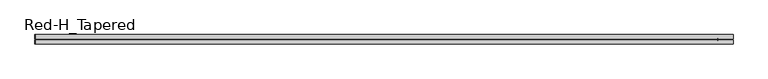
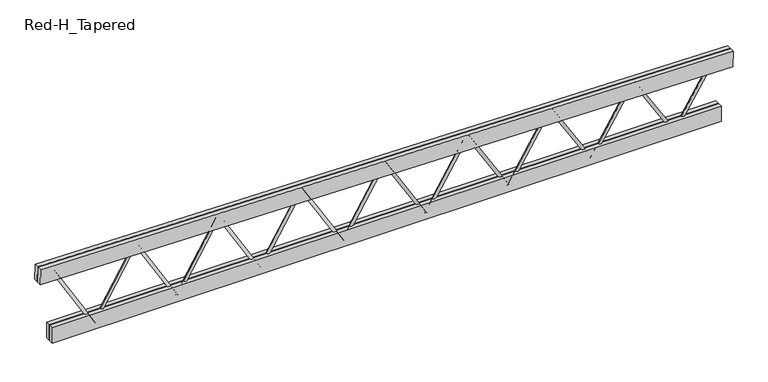
"""IFC4 building model written with IfcOpenShell, lengths in millimetres: beam geometry, Construction_Frames_RedBuilt_Openweb_Red-H_Tapered : Red-H_Tapered."""

from ifc_helpers import new_model, si_unit, point, frame, origin, origin_2d, place, context, project, spatial, polyline, circle_curve, trimmed, segment, composite_curve, outline, extrude, source, transform, mapped, element, save


def red_h_tapered_6d79e80b(model_context):
    return source(origin(), model_context, "Body", "SweptSolid", [
        extrude(outline(composite_curve([segment(trimmed(circle_curve(origin_2d(), 12.7), [point((0.0, 12.7))], [point((0.0, -12.7))], False, "CARTESIAN"), True, "CONTINUOUS"), segment(trimmed(circle_curve(origin_2d(), 12.7), [point((0.0, -12.7))], [point((0.0, 12.7))], False, "CARTESIAN"), True, "CONTINUOUS")], self_intersect=False)), frame((2526.107324, 0.0, -367.0101562), z_axis=(0.5255382750472374, 0.0, 0.8507699580147235), x_axis=(0.0, -1.0, 0.0)), (0.0, 0.0, 1.0), 686.6721074),
        extrude(outline(composite_curve([segment(trimmed(circle_curve(origin_2d(), 12.7), [point((0.0, -12.7))], [point((0.0, 12.6999999))], False, "CARTESIAN"), True, "CONTINUOUS"), segment(trimmed(circle_curve(origin_2d(), 12.7), [point((0.0, 12.6999999))], [point((0.0, -12.7))], False, "CARTESIAN"), True, "CONTINUOUS")], self_intersect=False)), frame((2526.107324, 0.0, -367.0101562), z_axis=(-0.5229651633515324, 0.0, 0.8523540566693545), x_axis=(0.0, -1.0, 0.0)), (0.0, 0.0, 1.0), 690.0506958),
        extrude(outline(composite_curve([segment(trimmed(circle_curve(origin_2d(), 12.7), [point((0.0, 12.7))], [point((0.0, -12.6999999))], False, "CARTESIAN"), True, "CONTINUOUS"), segment(trimmed(circle_curve(origin_2d(), 12.7), [point((0.0, -12.6999999))], [point((0.0, 12.7))], False, "CARTESIAN"), True, "CONTINUOUS")], self_intersect=False)), frame((1804.3623743, 0.0, -367.0101562), z_axis=(0.5229651633515339, 0.0, 0.8523540566693536), x_axis=(0.0, -1.0, 0.0)), (0.0, 0.0, 1.0), 690.0506958),
        extrude(outline(composite_curve([segment(trimmed(circle_curve(origin_2d(), 12.7), [point((0.0, -12.7000001))], [point((0.0, 12.6999999))], False, "CARTESIAN"), True, "CONTINUOUS"), segment(trimmed(circle_curve(origin_2d(), 12.7), [point((0.0, 12.6999999))], [point((0.0, -12.7000001))], False, "CARTESIAN"), True, "CONTINUOUS")], self_intersect=False)), frame((1804.3623743, 0.0, -367.0101562), z_axis=(-0.5204124432875953, 0.0, 0.8539150360963529), x_axis=(0.0, -1.0, 0.0)), (0.0, 0.0, 1.0), 693.4355231),
        extrude(outline(composite_curve([segment(trimmed(circle_curve(origin_2d(), 12.7), [point((0.0, 12.7))], [point((0.0, -12.7))], False, "CARTESIAN"), True, "CONTINUOUS"), segment(trimmed(circle_curve(origin_2d(), 12.7), [point((0.0, -12.7))], [point((0.0, 12.7))], False, "CARTESIAN"), True, "CONTINUOUS")], self_intersect=False)), frame((1082.6174246, 0.0, -367.0101562), z_axis=(0.5204124432875943, 0.0, 0.8539150360963534), x_axis=(0.0, -1.0, 0.0)), (0.0, 0.0, 1.0), 693.4355231),
        extrude(outline(composite_curve([segment(trimmed(circle_curve(origin_2d(), 12.7), [point((0.0, -12.7000001))], [point((0.0, 12.7))], False, "CARTESIAN"), True, "CONTINUOUS"), segment(trimmed(circle_curve(origin_2d(), 12.7), [point((0.0, 12.7))], [point((0.0, -12.7000001))], False, "CARTESIAN"), True, "CONTINUOUS")], self_intersect=False)), frame((1082.6174246, 0.0, -367.0101562), z_axis=(-0.5178799538342008, 0.0, 0.855453302884901), x_axis=(0.0, -1.0, 0.0)), (0.0, 0.0, 1.0), 696.8264985),
        extrude(outline(composite_curve([segment(trimmed(circle_curve(origin_2d(), 12.7), [point((0.0, 12.7))], [point((0.0, -12.7))], False, "CARTESIAN"), True, "CONTINUOUS"), segment(trimmed(circle_curve(origin_2d(), 12.7), [point((0.0, -12.7))], [point((0.0, 12.7))], False, "CARTESIAN"), True, "CONTINUOUS")], self_intersect=False)), frame((360.8724749, 0.0, -367.0101562), z_axis=(0.5178799538342008, 0.0, 0.855453302884901), x_axis=(0.0, -1.0, 0.0)), (0.0, 0.0, 1.0), 696.8264985),
        extrude(outline(composite_curve([segment(trimmed(circle_curve(origin_2d(), 12.7), [point((0.0, -12.7000001))], [point((0.0, 12.6999999))], False, "CARTESIAN"), True, "CONTINUOUS"), segment(trimmed(circle_curve(origin_2d(), 12.7), [point((0.0, 12.6999999))], [point((0.0, -12.7000001))], False, "CARTESIAN"), True, "CONTINUOUS")], self_intersect=False)), frame((360.8724749, 0.0, -367.0101562), z_axis=(-0.5153675335242818, 0.0, 0.856969255801571), x_axis=(0.0, -1.0, 0.0)), (0.0, 0.0, 1.0), 700.2235325),
        extrude(outline(composite_curve([segment(trimmed(circle_curve(origin_2d(), 12.7), [point((0.0, -12.6999999))], [point((0.0, 12.7000001))], False, "CARTESIAN"), True, "CONTINUOUS"), segment(trimmed(circle_curve(origin_2d(), 12.7), [point((0.0, 12.7000001))], [point((0.0, -12.6999999))], False, "CARTESIAN"), True, "CONTINUOUS")], self_intersect=False)), frame((-360.8724749, 0.0, -367.0101562), z_axis=(0.5153675335242504, 0.0, 0.8569692558015899), x_axis=(0.0, -1.0, 0.0)), (0.0, 0.0, 1.0), 700.2235325),
        extrude(outline(composite_curve([segment(trimmed(circle_curve(origin_2d(), 12.7), [point((0.0, 12.7))], [point((0.0, -12.7))], False, "CARTESIAN"), True, "CONTINUOUS"), segment(trimmed(circle_curve(origin_2d(), 12.7), [point((0.0, -12.7))], [point((0.0, 12.7))], False, "CARTESIAN"), True, "CONTINUOUS")], self_intersect=False)), frame((-360.8724749, 0.0, -367.0101562), z_axis=(-0.5128750205463383, 0.0, 0.8584632859357428), x_axis=(0.0, -1.0, 0.0)), (0.0, 0.0, 1.0), 703.6265375),
        extrude(outline(composite_curve([segment(trimmed(circle_curve(origin_2d(), 12.7), [point((0.0, -12.6999999))], [point((0.0, 12.7000001))], False, "CARTESIAN"), True, "CONTINUOUS"), segment(trimmed(circle_curve(origin_2d(), 12.7), [point((0.0, 12.7000001))], [point((0.0, -12.6999999))], False, "CARTESIAN"), True, "CONTINUOUS")], self_intersect=False)), frame((-1082.6174246, 0.0, -367.0101562), z_axis=(0.5128750205463365, 0.0, 0.858463285935744), x_axis=(0.0, -1.0, 0.0)), (0.0, 0.0, 1.0), 703.6265375),
        extrude(outline(composite_curve([segment(trimmed(circle_curve(origin_2d(), 12.7), [point((0.0, 12.7))], [point((0.0, -12.7))], False, "CARTESIAN"), True, "CONTINUOUS"), segment(trimmed(circle_curve(origin_2d(), 12.7), [point((0.0, -12.7))], [point((0.0, 12.7))], False, "CARTESIAN"), True, "CONTINUOUS")], self_intersect=False)), frame((-1082.6174246, 0.0, -367.0101562), z_axis=(-0.5104022528410607, 0.0, 0.8599357768431141), x_axis=(0.0, -1.0, 0.0)), (0.0, 0.0, 1.0), 707.0354272),
        extrude(outline(composite_curve([segment(trimmed(circle_curve(origin_2d(), 12.7), [point((0.0, -12.7))], [point((0.0, 12.7000001))], False, "CARTESIAN"), True, "CONTINUOUS"), segment(trimmed(circle_curve(origin_2d(), 12.7), [point((0.0, 12.7000001))], [point((0.0, -12.7))], False, "CARTESIAN"), True, "CONTINUOUS")], self_intersect=False)), frame((-1804.3623743, 0.0, -367.0101562), z_axis=(0.510402252841074, 0.0, 0.8599357768431061), x_axis=(0.0, -1.0, 0.0)), (0.0, 0.0, 1.0), 707.0354272),
        extrude(outline(composite_curve([segment(trimmed(circle_curve(origin_2d(), 12.7), [point((0.0, 12.6999999))], [point((0.0, -12.7))], False, "CARTESIAN"), True, "CONTINUOUS"), segment(trimmed(circle_curve(origin_2d(), 12.7), [point((0.0, -12.7))], [point((0.0, 12.6999999))], False, "CARTESIAN"), True, "CONTINUOUS")], self_intersect=False)), frame((-1804.3623743, 0.0, -367.0101562), z_axis=(-0.5079490681928376, 0.0, 0.8613871046875662), x_axis=(0.0, -1.0, 0.0)), (0.0, 0.0, 1.0), 710.4501169),
        extrude(outline(composite_curve([segment(trimmed(circle_curve(origin_2d(), 12.7), [point((0.0, -12.6999999))], [point((0.0, 12.7))], False, "CARTESIAN"), True, "CONTINUOUS"), segment(trimmed(circle_curve(origin_2d(), 12.7), [point((0.0, 12.7))], [point((0.0, -12.6999999))], False, "CARTESIAN"), True, "CONTINUOUS")], self_intersect=False)), frame((-2526.107324, 0.0, -367.0101562), z_axis=(0.5079490681928277, 0.0, 0.861387104687572), x_axis=(0.0, -1.0, 0.0)), (0.0, 0.0, 1.0), 710.4501169),
        extrude(outline(composite_curve([segment(trimmed(circle_curve(origin_2d(), 12.7), [point((0.0, 12.7))], [point((0.0, -12.7))], False, "CARTESIAN"), True, "CONTINUOUS"), segment(trimmed(circle_curve(origin_2d(), 12.7), [point((0.0, -12.7))], [point((0.0, 12.7))], False, "CARTESIAN"), True, "CONTINUOUS")], self_intersect=False)), frame((-2526.107324, 0.0, -367.0101562), z_axis=(-0.5055153043168177, 0.0, 0.8628176383810633), x_axis=(0.0, -1.0, 0.0)), (0.0, 0.0, 1.0), 713.8705234),
        extrude(outline(polyline([(-2912.3797989, -41.275), (-2912.3797989, -3.175), (2912.3797989, -3.175), (2912.3797989, -41.275), (-2912.3797989, -41.275)])), frame((0.0, 0.0, -386.0601562), z_axis=(0.0, 0.0, 1.0), x_axis=(1.0, 0.0, 0.0)), (0.0, 0.0, 1.0), 139.7),
        extrude(outline(polyline([(-2912.3797989, 3.175), (-2912.3797989, 41.275), (2912.3797989, 41.275), (2912.3797989, 3.175), (-2912.3797989, 3.175)])), frame((0.0, 0.0, -386.0601562), z_axis=(0.0, 0.0, 1.0), x_axis=(1.0, 0.0, 0.0)), (0.0, 0.0, 1.0), 139.7),
        extrude(outline(polyline([(0.0, -38.1), (0.0, 0.0), (6028.8157603, 0.0), (6028.8157603, -38.1), (0.0, -38.1)])), frame((-3016.3340788, -3.175, 185.4596828), z_axis=(0.016852397558582144, 0.0, 0.9998579882645973), x_axis=(0.9998579882645973, 0.0, -0.016852397558582144)), (0.0, 0.0, 1.0), 139.7),
        extrude(outline(polyline([(0.0, -38.1), (0.0, 0.0), (6028.8157603, 0.0), (6028.8157603, -38.1), (0.0, -38.1)])), frame((-3016.3340788, 41.275, 185.4596828), z_axis=(0.016852397558582144, 0.0, 0.9998579882645973), x_axis=(0.9998579882645973, 0.0, -0.016852397558582144)), (0.0, 0.0, 1.0), 139.7),
    ])


if __name__ == "__main__":
    model = new_model("IFC4")
    model_context = context("Model", 3, world=origin())
    ifc_project = project(units=[si_unit("LENGTHUNIT", "METRE", prefix="MILLI")], contexts=[model_context])
    site = spatial("IfcSite", under=ifc_project)
    building = spatial("IfcBuilding", under=site)
    placement = place(None, origin())
    red_h_tapered_shape = red_h_tapered_6d79e80b(model_context)
    element("IfcBeam", 1, ObjectType="Construction_Frames_RedBuilt_Openweb_Red-H_Tapered : Red-H_Tapered", at=placement, inside=building, context=model_context, shape_type="MappedRepresentation", body=[
        mapped(red_h_tapered_shape, transform((0.0, 0.0, 0.0), x_axis=(1.0, 0.0, 0.0), y_axis=(0.0, 1.0, 0.0), z_axis=(0.0, 0.0, 1.0))),
    ])
    save(model, "model.ifc")

# Revit data of these elements
# Type "Construction_Frames_RedBuilt_Openweb_Red-H_Tapered : Red-H_Tapered"
#   Youtube clip = ""
#   Weight Net (Kg) = "0"
#   Webs = "Up to 2\" diameter tubular steel"
#   Uniformat II Description = ""
#   Uniformat II Code = ""
#   Uniclass 2015 Name = "Softwood trusses"
#   Uniclass 2015 Code = "Pr_20_85_90_81"
#   Uniclass 2.0 Description = "Structural Framing Systems"
#   Uniclass 2.0 Code = "SS-15-10-75"
#   Uniclass 1.4 Description = "Trusses"
#   Uniclass 1.4 Code = "L3523"
#   UNSPSC Code = "30103606"
#   Technical description = "http://www.redbuilt.com/reference/literature-and-other-resources"
#   Region South America = "None"
#   Region Oceania = "None"
#   Region North America = "US"
#   Region Middle East = "None"
#   Region Europe = "None"
#   Region Asia = "None"
#   Region Antarctica = "None"
#   Region Africa = "None"
#   QR code = "http://bimobject.com/redbuilt/product/redbuilt-0003"
#   Product url = "http://www.redbuilt.com/products/default.aspx?id=2"
#   Product group = "Wood Trusses"
#   Product family = "Construction"
#   Product data url = "https://bimobject.com/redbuilt/product/redbuilt-0003"
#   Product certification = ""
#   Product SKU = "redbuilt-0003"
#   Product Page URL = "http://www.redbuilt.com/commercial-systems/red-m-red-h-open-web-trusses"
#   Product Guid = "2c5793f2-6ffb-4665-b825-cf90c048e711"
#   Product Documentation Link = "http://www.redbuilt.com/documents/OW_Guide_2017_07_LowRes_wLinks.pdf"
#   OmniClass Description = "Wood Trusses"
#   OmniClass Code = "23-13 35 19 13 17"
#   NBS Reference Description = ""
#   NBS Reference Code = ""
#   Material secondary = "Steel"
#   Material main = "CHARRED WOOD"
#   Masterformat 2014 Description = "Metal-Web Wood Joists"
#   Masterformat 2014 Code = "06 17 36"
#   Manufacturer name = "RedBuilt"
#   Manufacturer country = "United States"
#   Installation instructions = "http://www.redbuilt.com/documents/Installation_Sheets_Open-Web.pdf"
#   IFC Classification = ""
#   EAN code = ""
#   Design country = "United States"
#   Product Information = "http://redbuilt.com/products/default.aspx?id=2"
#   Model = "Red-H-Tapered"
#   Manufacturer URL = "http://redbuilt.com/"
#   Manufacturer = "RedBuilt™"
#   Description = "Open Web Truss"
#   Date of publishing = "8/17/2010"
#   Contact us = "http://redbuilt.com/contact/"
#   Chords = "Double 1½\" x 5½\" MSR lumber"
#   COBIe Type Category = ""
#   Brand url = "http://www.redbuilt.com"
#   BIMobject main category code = "construction"
#   BIMobject main category = "Construction"
#   BIMobject category code = "construction-frames-trusses"
#   BIMobject category = "Frames & Trusses"
#   Web Radius = 0' - 0 1/2"
#   Web Layout Offset Start [instance default] = 0' - 5"
#   Web Layout Offset End [instance default] = 0' - 5"
#   Web Diameter = 0' - 1"
#   TotalLength [instance default] = 20' - 0"
#   Span Minimum = 4' - 0"
#   Span Maximum = 70' - 0"
#   Span Limit [instance default] = 20' - 0"
#   Nominal width = 0' - 0"
#   Nominal height = 0' - 0"
#   Inner Depth Top [instance default] = 0' - 2.76372"
#   Depth Start [instance default] = 6' - 0"
#   Top Chord Length [instance default] = 20' - 1.19701"
#   TC Extension Start Aux [instance default] = 0' - 0"
#   TC Extension End Aux [instance default] = 0' - 0"
#   T-B Chord Length Difference L [instance default] = 0' - 4"
#   T-B Chord Length Difference [instance default] = 0' - 4"
#   Height 2 [instance default] = 6' - 0"
#   Depth Minimum at Wall = 2' - 0"
#   Depth Maximum at Wall = 6' - 0"
#   Depth Lower End [instance default] = 2' - 0"
#   Depth Higher End [instance default] = 6' - 0"
#   Depth End [instance default] = 2' - 0"
#   Depth 2 [instance default] = 2' - 0"
#   Chord Width = 0' - 3 1/4"
#   Chord Thickness = 0' - 1 1/2"
#   Chord Depth = 0' - 5 1/2"
#   Offset Start [instance default] = 0' - 0"
#   TC Extension Start [instance default] = 0' - 0"
#   End Panel = 0' - 5"
#   Offset End [instance default] = 0' - 0"
#   TC Extension End [instance default] = 0' - 0"
#   Length [instance default] = 20' - 0"
#   Angle [instance default] = 5.71059°
#   Span Limit Warning [instance default] = no
#   Edition number = 1
#   Top Bearing Start [instance default] = yes
#   Top Bearing End [instance default] = yes
#   Bottom Bearing Start [instance default] = no
#   Bottom Bearing End [instance default] = no
#   8 Panels [instance default] = yes
#   16 Panels [instance default] = no
#   12 Panels [instance default] = no
#   Web Material = RedBuilt-Steel, Galvanized
#   Clip Material = RedBuilt-Steel, Galvanized
#   Chords Material = WOOD-OAKFIRE
#   URL = ""
#   Assembly Code = ""
# Element 1 (IfcBeam, "Construction_Frames_RedBuilt_Openweb_Red-H_Tapered : Red-H_Tapered")
#   TotalLength = 19' - 9.32124"
#   Span Limit = 19' - 9.32124"
#   Inner Depth Top = 0' - 2.75039"
#   Depth Start = 5' - 0"
#   Top Chord Length = 19' - 9.35495"
#   Height 2 = 5' - 0"
#   Depth Higher End = 5' - 0"
#   Depth 2 = 0' - 4"
#   Angle = 0.965617°
#   Materials on its faces: "RedBuilt-Steel, Galvanized", "WOOD-OAKFIRE"
# Materials
#   "RedBuilt-Steel, Galvanized": class "Metal", colour RGB 164 172 176, transparency 0, Manufacturer = "RedBuilt. LLC", Comments = "Openweb Metal Web", URL = "http://www.redbuilt.com/", Description = "Galvanized steel", Cost = 0
#   "WOOD-OAKFIRE": class "Wood", colour RGB 198 202 183, transparency 0, Description = "Generic wood", Cost = 0
